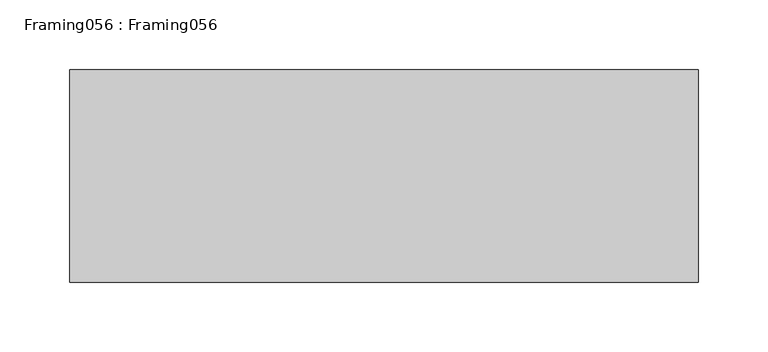
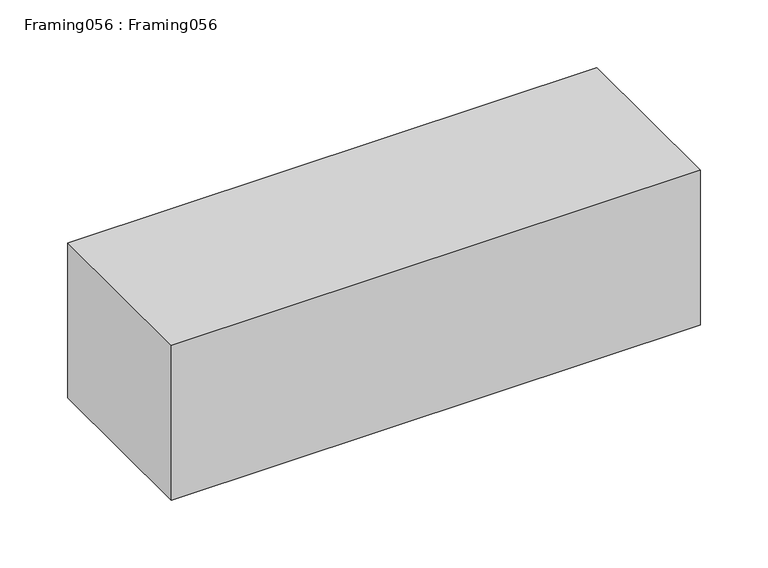
"""IFC4 building model written with IfcOpenShell, lengths in millimetres: proxy geometry, Framing056 : Framing056."""

from ifc_helpers import new_model, si_unit, frame, origin, place, context, project, spatial, polyline, outline, extrude, source, transform, mapped, element, save


def framing056_framing056_6f68aedc(model_context):
    return source(origin(), model_context, "Body", "SweptSolid", [
        extrude(outline(polyline([(-4474.0538825, 794.7093426), (-4924.9038825, 794.7093426), (-4924.9038825, 947.1093426), (-4474.0538825, 947.1093426), (-4474.0538825, 794.7093426)])), frame((0.0, 0.0, 39579.2960083), z_axis=(0.0, 0.0, 1.0), x_axis=(1.0, 0.0, 0.0)), (0.0, 0.0, 1.0), 139.7),
    ])


if __name__ == "__main__":
    model = new_model("IFC4")
    model_context = context("Model", 3, world=origin())
    ifc_project = project(units=[si_unit("LENGTHUNIT", "METRE", prefix="MILLI")], contexts=[model_context])
    site = spatial("IfcSite", under=ifc_project)
    building = spatial("IfcBuilding", under=site)
    placement = place(None, origin())
    framing056_framing056_shape = framing056_framing056_6f68aedc(model_context)
    element("IfcBuildingElementProxy", 1, Name="Framing056 : Framing056", ObjectType="Framing056 : Framing056", at=placement, inside=building, context=model_context, shape_type="MappedRepresentation", body=[
        mapped(framing056_framing056_shape, transform((0.0, 0.0, 0.0), x_axis=(1.0, 0.0, 0.0), y_axis=(0.0, 1.0, 0.0), z_axis=(0.0, 0.0, 1.0))),
    ])
    save(model, "model.ifc")

# Revit data of these elements
# Type "Framing056 : Framing056"
#   NameOverride = "Framing056"
# Element 1 (IfcBuildingElementProxy, "Framing056 : Framing056")
#   Materials on its faces: "WOOD FRAMING (SEE STRUCT DWGS)"
# Materials
#   "WOOD FRAMING (SEE STRUCT DWGS)": class "Unassigned", colour RGB 224 188 168, transparency 0, Cost = 0
